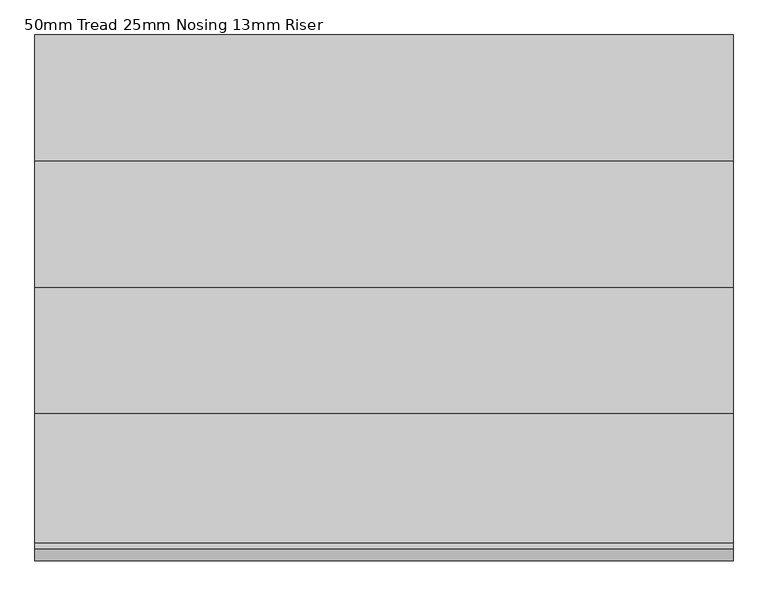
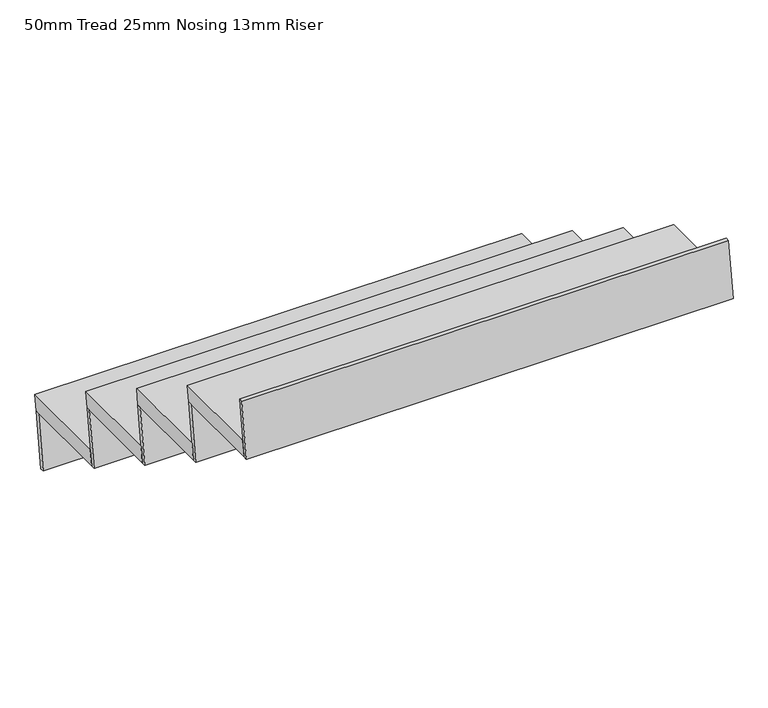
"""IFC4 building model written with IfcOpenShell, lengths in millimetres: stair flight geometry, 50mm Tread 25mm Nosing 13mm Riser."""

from ifc_helpers import new_model, si_unit, frame, origin, place, context, project, spatial, polyline, outline, extrude, source, transform, mapped, element, save


def stair_flight_50mm_tread_25mm_nosing_13mm_riser_53dc4827(model_context):
    return source(origin(), model_context, "Body", "SweptSolid", [
        extrude(outline(polyline([(7032.4781803, 8794.1176471), (7332.4781803, 8794.1176471), (7325.3948469, 8744.1176471), (7025.3948469, 8744.1176471), (7032.4781803, 8794.1176471)])), frame((-226.7120949, 0.0, 0.0), z_axis=(1.0, 0.0, 0.0), x_axis=(0.0, 1.0, 0.0)), (0.0, 0.0, 1.0), 1520.0),
        extrude(outline(polyline([(7325.3948469, 8744.1176471), (7300.3948469, 8567.6470588), (7287.770036, 8567.6470588), (7312.770036, 8744.1176471), (7325.3948469, 8744.1176471)])), frame((-226.7120949, 0.0, 0.0), z_axis=(1.0, 0.0, 0.0), x_axis=(0.0, 1.0, 0.0)), (0.0, 0.0, 1.0), 1520.0),
        extrude(outline(polyline([(7050.3948469, 8920.5882353), (7025.3948469, 8744.1176471), (7012.770036, 8744.1176471), (7037.770036, 8920.5882353), (7050.3948469, 8920.5882353)])), frame((-226.7120949, 0.0, 0.0), z_axis=(1.0, 0.0, 0.0), x_axis=(0.0, 1.0, 0.0)), (0.0, 0.0, 1.0), 1520.0),
        extrude(outline(polyline([(6757.4781803, 8970.5882353), (7057.4781803, 8970.5882353), (7050.3948469, 8920.5882353), (6750.3948469, 8920.5882353), (6757.4781803, 8970.5882353)])), frame((-226.7120949, 0.0, 0.0), z_axis=(1.0, 0.0, 0.0), x_axis=(0.0, 1.0, 0.0)), (0.0, 0.0, 1.0), 1520.0),
        extrude(outline(polyline([(6775.3948469, 9097.0588235), (6750.3948469, 8920.5882353), (6737.770036, 8920.5882353), (6762.770036, 9097.0588235), (6775.3948469, 9097.0588235)])), frame((-226.7120949, 0.0, 0.0), z_axis=(1.0, 0.0, 0.0), x_axis=(0.0, 1.0, 0.0)), (0.0, 0.0, 1.0), 1520.0),
        extrude(outline(polyline([(6482.4781803, 9147.0588235), (6782.4781803, 9147.0588235), (6775.3948469, 9097.0588235), (6475.3948469, 9097.0588235), (6482.4781803, 9147.0588235)])), frame((-226.7120949, 0.0, 0.0), z_axis=(1.0, 0.0, 0.0), x_axis=(0.0, 1.0, 0.0)), (0.0, 0.0, 1.0), 1520.0),
        extrude(outline(polyline([(6500.3948469, 9273.5294118), (6475.3948469, 9097.0588235), (6462.770036, 9097.0588235), (6487.770036, 9273.5294118), (6500.3948469, 9273.5294118)])), frame((-226.7120949, 0.0, 0.0), z_axis=(1.0, 0.0, 0.0), x_axis=(0.0, 1.0, 0.0)), (0.0, 0.0, 1.0), 1520.0),
        extrude(outline(polyline([(6225.3948469, 9450.0), (6200.3948469, 9273.5294118), (6187.770036, 9273.5294118), (6212.770036, 9450.0), (6225.3948469, 9450.0)])), frame((-226.7120949, 0.0, 0.0), z_axis=(1.0, 0.0, 0.0), x_axis=(0.0, 1.0, 0.0)), (0.0, 0.0, 1.0), 1520.0),
        extrude(outline(polyline([(6207.4781803, 9323.5294118), (6507.4781803, 9323.5294118), (6500.3948469, 9273.5294118), (6200.3948469, 9273.5294118), (6207.4781803, 9323.5294118)])), frame((-226.7120949, 0.0, 0.0), z_axis=(1.0, 0.0, 0.0), x_axis=(0.0, 1.0, 0.0)), (0.0, 0.0, 1.0), 1520.0),
    ])


if __name__ == "__main__":
    model = new_model("IFC4")
    model_context = context("Model", 3, world=origin())
    ifc_project = project(units=[si_unit("LENGTHUNIT", "METRE", prefix="MILLI")], contexts=[model_context])
    site = spatial("IfcSite", under=ifc_project)
    building = spatial("IfcBuilding", under=site)
    placement = place(None, origin())
    stair_flight_50mm_tread_25mm_nosing_13mm_riser_shape = stair_flight_50mm_tread_25mm_nosing_13mm_riser_53dc4827(model_context)
    element("IfcStairFlight", 1, ObjectType="50mm Tread 25mm Nosing 13mm Riser", at=placement, inside=building, context=model_context, shape_type="MappedRepresentation", body=[
        mapped(stair_flight_50mm_tread_25mm_nosing_13mm_riser_shape, transform((0.0, 0.0, 0.0), x_axis=(1.0, 0.0, 0.0), y_axis=(0.0, 1.0, 0.0), z_axis=(0.0, 0.0, 1.0))),
    ])
    save(model, "model.ifc")
